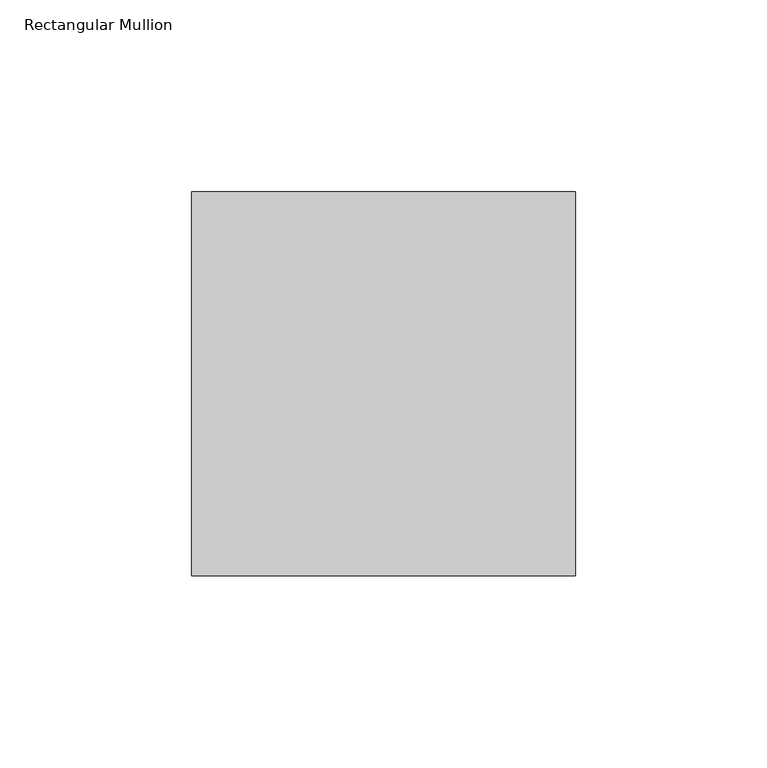
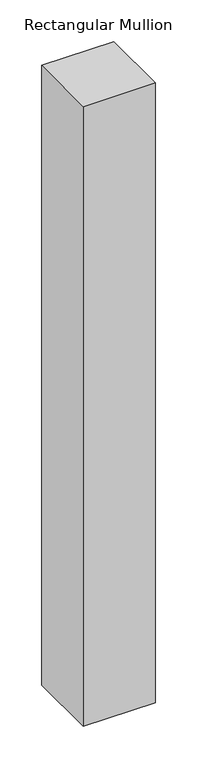
"""IFC4 building model written with IfcOpenShell, lengths in millimetres: member geometry, Rectangular Mullion : 알루미늄_Rectangular Cap_100 x100."""

import ifcopenshell
import ifcopenshell.guid

model = None  # the IFC model being written
_history = None  # IfcOwnerHistory: only IFC2X3 demands one
_inside = {}  # id of a spatial element -> (the spatial element, [elements in it])
_under = {}  # id of a project, library or spatial element -> (it, [spatial elements below it])
_declared = {}  # id of a project -> (the project, [libraries it declares])
_typed = {}  # id of a type object -> (the type object, [elements of that type])
_made_of = {}  # id of a material, layer set ... -> (it, [elements and type objects made of it])


def new_model(schema):
    """Start an empty IFC model of exactly this schema.

    Asked for "IFC4X3", IfcOpenShell would pick the latest addendum, in which some entities
    have other attributes; the version numbers below select the first issue.
    IFC2X3 requires an IfcOwnerHistory on every rooted entity: one is made here for all.
    """
    global model, _history
    if schema == "IFC4X3":
        model = ifcopenshell.file(schema_version=(4, 3, 0, 0))
    else:
        model = ifcopenshell.file(schema=schema)
    _inside.clear()
    _under.clear()
    _declared.clear()
    _typed.clear()
    _made_of.clear()
    _history = None
    if model.schema == "IFC2X3":
        org = make("IfcOrganization", Name="unknown")
        user = make(
            "IfcPersonAndOrganization",
            ThePerson=make("IfcPerson", FamilyName="unknown"),
            TheOrganization=org,
        )
        app = make(
            "IfcApplication",
            ApplicationDeveloper=org,
            Version="unknown",
            ApplicationFullName="unknown",
            ApplicationIdentifier="unknown",
        )
        _history = make(
            "IfcOwnerHistory",
            OwningUser=user,
            OwningApplication=app,
            ChangeAction="ADDED",
            CreationDate=0,
        )
    return model


def make(cls, **values):
    """One entity of the class cls with the attributes given. An attribute that is None is left unset."""
    return model.create_entity(
        cls, **{name: value for name, value in values.items() if value is not None}
    )


def rooted(cls, **values):
    """An entity with a GlobalId (a new one), such as an element, a storey or a relation."""
    return make(cls, GlobalId=ifcopenshell.guid.new(), OwnerHistory=_history, **values)


def si_unit(unit_type, name, prefix=None):
    """IfcSIUnit, for example si_unit("LENGTHUNIT", "METRE", prefix="MILLI")."""
    return make("IfcSIUnit", UnitType=unit_type, Prefix=prefix, Name=name)


def assignment(units):
    """IfcUnitAssignment: the units of a project."""
    return None if units is None else make("IfcUnitAssignment", Units=units)


def point(xyz):
    """IfcCartesianPoint."""
    return None if xyz is None else make("IfcCartesianPoint", Coordinates=xyz)


def direction(xyz):
    """IfcDirection."""
    return None if xyz is None else make("IfcDirection", DirectionRatios=xyz)


def frame(location, z_axis=None, x_axis=None):
    """IfcAxis2Placement3D, a coordinate frame: its origin and axes. An axis left out is left unset."""
    return make(
        "IfcAxis2Placement3D",
        Location=point(location),
        Axis=direction(z_axis),
        RefDirection=direction(x_axis),
    )


def origin():
    """The frame at (0, 0, 0) with its axes left unset."""
    return frame((0.0, 0.0, 0.0))


def place(relative_to, where):
    """IfcLocalPlacement: puts the frame where relative to a parent placement (None: the world)."""
    return make(
        "IfcLocalPlacement", PlacementRelTo=relative_to, RelativePlacement=where
    )


def context(
    kind, dimensions, precision=None, world=None, true_north=None, identifier=None
):
    """IfcGeometricRepresentationContext, for example the 3D "Model" context."""
    return make(
        "IfcGeometricRepresentationContext",
        ContextIdentifier=identifier,
        ContextType=kind,
        CoordinateSpaceDimension=dimensions,
        Precision=precision,
        WorldCoordinateSystem=world,
        TrueNorth=true_north,
    )


def project(units=None, contexts=None):
    """IfcProject with its units and contexts."""
    return rooted(
        "IfcProject",
        Name="project",
        RepresentationContexts=contexts,
        UnitsInContext=assignment(units),
    )


def spatial(cls, under=None, at=None, **own):
    """A site, building, storey or space (cls), placed at a placement, below another one or the project."""
    s = rooted(cls, ObjectPlacement=at, **own)
    if under is not None:
        _under.setdefault(under.id(), (under, []))[1].append(s)
    return s


def polyline(points):
    """IfcPolyline through the points."""
    return make("IfcPolyline", Points=[point(p) for p in points])


def outline(outer, holes=None, kind="AREA"):
    """IfcArbitraryClosedProfileDef: a profile drawn as a closed curve; with holes, ...WithVoids."""
    if holes is None:
        return make("IfcArbitraryClosedProfileDef", ProfileType=kind, OuterCurve=outer)
    return make(
        "IfcArbitraryProfileDefWithVoids",
        ProfileType=kind,
        OuterCurve=outer,
        InnerCurves=holes,
    )


def extrude(swept, where, along, depth):
    """IfcExtrudedAreaSolid: the profile swept, set in the frame where, extruded along a direction by depth."""
    return make(
        "IfcExtrudedAreaSolid",
        SweptArea=swept,
        Position=where,
        ExtrudedDirection=direction(along),
        Depth=depth,
    )


def shape(context_of_items, identifier, shape_type, items):
    """IfcShapeRepresentation: the items that make up one representation, for example the "Body"."""
    return make(
        "IfcShapeRepresentation",
        ContextOfItems=context_of_items,
        RepresentationIdentifier=identifier,
        RepresentationType=shape_type,
        Items=items,
    )


def source(mapping_origin, context_of_items, identifier, shape_type, items):
    """IfcRepresentationMap: a shape defined once, which mapped items show again and again."""
    return make(
        "IfcRepresentationMap",
        MappingOrigin=mapping_origin,
        MappedRepresentation=shape(context_of_items, identifier, shape_type, items),
    )


def transform(
    local_origin,
    x_axis=None,
    y_axis=None,
    z_axis=None,
    scale=None,
    scale2=None,
    scale3=None,
    uniform=True,
):
    """IfcCartesianTransformationOperator3D, or its non-uniform kind. x_axis, y_axis, z_axis: its Axis1, 2, 3."""
    if uniform:
        return make(
            "IfcCartesianTransformationOperator3D",
            Axis1=direction(x_axis),
            Axis2=direction(y_axis),
            LocalOrigin=point(local_origin),
            Scale=scale,
            Axis3=direction(z_axis),
        )
    return make(
        "IfcCartesianTransformationOperator3DnonUniform",
        Axis1=direction(x_axis),
        Axis2=direction(y_axis),
        LocalOrigin=point(local_origin),
        Scale=scale,
        Axis3=direction(z_axis),
        Scale2=scale2,
        Scale3=scale3,
    )


def mapped(mapping_source, mapping_target):
    """IfcMappedItem: shows the shape of a source again, moved by a transform."""
    return make(
        "IfcMappedItem", MappingSource=mapping_source, MappingTarget=mapping_target
    )


def made_of(thing, what):
    """Note that an element or type object is made of a material, layer set ...; save() writes the relation."""
    if what is not None:
        _made_of.setdefault(what.id(), (what, []))[1].append(thing)
    return thing


def element(
    cls,
    number,
    at=None,
    inside=None,
    cuts=None,
    type_object=None,
    material=None,
    context=None,
    identifier="Body",
    shape_type=None,
    held_by="IfcProductDefinitionShape",
    body=None,
    shapes=None,
    **own,
):
    """One element of the class cls, such as IfcWall. Its Tag is "e" and its number.

    at: its placement. inside: the storey or other place that contains it. cuts: it is an
    opening in that element (IfcRelVoidsElement). A single representation is given by context,
    identifier, shape_type and body (its items); several are given by shapes. held_by: the class
    of the entity that holds the representations. save() writes the other relations.
    """
    e = rooted(cls, Tag="e%d" % number, ObjectPlacement=at, **own)
    if body is not None:
        shapes = [shape(context, identifier, shape_type, body)]
    if shapes is not None:
        e.Representation = make(held_by, Representations=shapes)
    if inside is not None:
        _inside.setdefault(inside.id(), (inside, []))[1].append(e)
    if cuts is not None:
        rooted(
            "IfcRelVoidsElement", RelatingBuildingElement=cuts, RelatedOpeningElement=e
        )
    if type_object is not None:
        _typed.setdefault(type_object.id(), (type_object, []))[1].append(e)
    return made_of(e, material)


def aggregate(whole, parts):
    """IfcRelAggregates: a whole, such as a stair, and the parts it consists of."""
    return rooted("IfcRelAggregates", RelatingObject=whole, RelatedObjects=parts)


def save(model, path):
    """Write the relations noted so far, then the file.

    IfcRelAggregates (storeys below a building ...), IfcRelContainedInSpatialStructure (elements
    in a storey), IfcRelDefinesByType, IfcRelAssociatesMaterial and IfcRelDeclares: one each for
    every whole, place, type object, material and project.
    """
    for whole, parts in _under.values():
        aggregate(whole, parts)
    for where, things in _inside.values():
        rooted(
            "IfcRelContainedInSpatialStructure",
            RelatedElements=things,
            RelatingStructure=where,
        )
    for kind, things in _typed.values():
        rooted("IfcRelDefinesByType", RelatedObjects=things, RelatingType=kind)
    for what, things in _made_of.values():
        rooted("IfcRelAssociatesMaterial", RelatedObjects=things, RelatingMaterial=what)
    for by, libraries in _declared.values():
        rooted("IfcRelDeclares", RelatingContext=by, RelatedDefinitions=libraries)
    model.write(path)


def rectangular_mullion_dadccf76(model_context):
    return source(origin(), model_context, "Body", "SweptSolid", [
        extrude(outline(polyline([(0.0, 50.0), (0.0, -50.0), (-100.0, -50.0), (-100.0, 50.0), (0.0, 50.0)])), frame((0.0, 0.0, -910.0), z_axis=(0.0, 0.0, 1.0), x_axis=(1.0, 0.0, 0.0)), (0.0, 0.0, 1.0), 910.0),
    ])


if __name__ == "__main__":
    model = new_model("IFC4")
    model_context = context("Model", 3, world=origin())
    ifc_project = project(units=[si_unit("LENGTHUNIT", "METRE", prefix="MILLI")], contexts=[model_context])
    site = spatial("IfcSite", under=ifc_project)
    building = spatial("IfcBuilding", under=site)
    placement = place(None, origin())
    rectangular_mullion_shape = rectangular_mullion_dadccf76(model_context)
    element("IfcMember", 1, ObjectType="Rectangular Mullion : 알루미늄_Rectangular Cap_100 x100", at=placement, inside=building, context=model_context, shape_type="MappedRepresentation", body=[
        mapped(rectangular_mullion_shape, transform((0.0, 0.0, 0.0), x_axis=(1.0, 0.0, 0.0), y_axis=(0.0, 1.0, 0.0), z_axis=(0.0, 0.0, 1.0))),
    ])
    save(model, "model.ifc")

# Revit data of these elements
# Type "Rectangular Mullion : 알루미늄_Rectangular Cap_100 x100"
#   built-in parameter 1007304 = 0.328084 (stored number, unit not read)
#   built-in parameter 1007301 = 0.164042 (stored number, unit not read)
#   built-in parameter 1007300 = 0.164042 (stored number, unit not read)
# Element 1 (IfcMember, "Rectangular Mullion : 알루미늄_Rectangular Cap_100 x100")
#   Materials on its faces: "00_Metal_Stainless Steel"
# Materials
#   "00_Metal_Stainless Steel": class "Metal", colour RGB 148 148 148, transparency 0, Description = "Steel", Cost = 0
